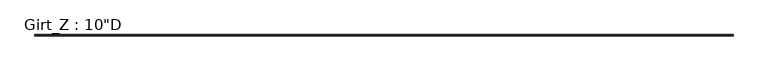
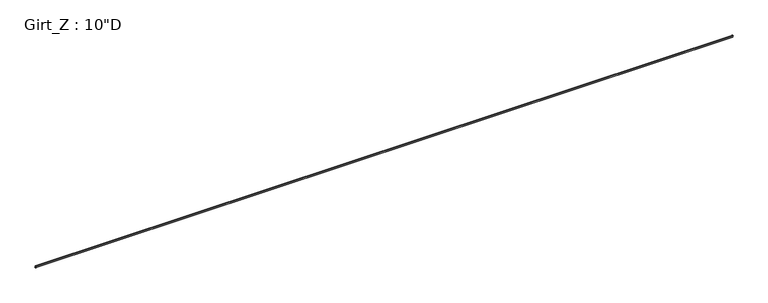
"""IFC4 building model written with IfcOpenShell, lengths in millimetres: beam geometry."""

from ifc_helpers import new_model, si_unit, point, frame, frame_2d, origin, place, context, project, spatial, polyline, circle_curve, trimmed, segment, composite_curve, outline, extrude, source, transform, mapped, element, save


def beam_261beed4(model_context):
    return source(origin(), model_context, "Body", "SweptSolid", [
        extrude(outline(composite_curve([segment(polyline([(-77.9859375, 127.0), (-3.3734375, 127.0)]), True, "CONTINUOUS"), segment(trimmed(circle_curve(frame_2d((-3.3734375, 122.2375)), 4.7625), [point((-3.3734375, 127.0))], [point((1.3890625, 122.2375))], False, "CARTESIAN"), True, "CONTINUOUS"), segment(polyline([(1.3890625, 122.2375), (1.3890625, -122.2389339)]), True, "CONTINUOUS"), segment(trimmed(circle_curve(frame_2d((3.3748024, -122.2389339)), 1.9857399), [point((1.3890625, -122.2389339))], [point((3.2694106, -124.221875))], True, "CARTESIAN"), True, "CONTINUOUS"), segment(polyline([(3.2694106, -124.221875), (83.0404765, -124.221875), (94.4528742, -110.621109), (96.5810415, -112.4068534), (84.3359375, -127.0), (-1.3890625, -127.0), (-1.3890625, 122.2381931)]), True, "CONTINUOUS"), segment(trimmed(circle_curve(frame_2d((-3.3741066, 122.2381931)), 1.9850441), [point((-1.3890625, 122.2381931))], [point((-3.3005807, 124.221875))], True, "CARTESIAN"), True, "CONTINUOUS"), segment(polyline([(-3.3005807, 124.221875), (-76.6904765, 124.221875), (-88.1028742, 110.621109), (-90.2310415, 112.4068534), (-77.9859375, 127.0)]), True, "CONTINUOUS")], self_intersect=False)), frame((-44323.0, 0.0, 0.0), z_axis=(1.0, 0.0, 0.0), x_axis=(0.0, 1.0, 0.0)), (0.0, 0.0, 1.0), 88430.1),
    ])


if __name__ == "__main__":
    model = new_model("IFC4")
    model_context = context("Model", 3, world=origin())
    ifc_project = project(units=[si_unit("LENGTHUNIT", "METRE", prefix="MILLI")], contexts=[model_context])
    site = spatial("IfcSite", under=ifc_project)
    building = spatial("IfcBuilding", under=site)
    placement = place(None, origin())
    beam_shape = beam_261beed4(model_context)
    element("IfcBeam", 1, ObjectType="Girt_Z : 10\"D", at=placement, inside=building, context=model_context, shape_type="MappedRepresentation", body=[
        mapped(beam_shape, transform((0.0, 0.0, 0.0), x_axis=(1.0, 0.0, 0.0), y_axis=(0.0, 1.0, 0.0), z_axis=(0.0, 0.0, 1.0))),
    ])
    save(model, "model.ifc")

# Revit data of these elements
# Type "Girt_Z : 10\"D"
#   half leg = 0' - 1 11/16"
#   Web_Thickness = 0' - 0 7/64"
#   Length [instance default] = 10' - 0"
#   Leg_2 = 0' - 3 3/8"
#   Leg_1 = 0' - 3 1/8"
#   Height = 0' - 10"
#   Structural Material [instance default] = none
# Element 1 (IfcBeam, "Girt_Z : 10\"D")
#   Structural Material = STRUCTURAL STEEL - SEE STRUCT. DWGS
#   Materials on its faces: "STRUCTURAL STEEL - SEE STRUCT. DWGS"
# Materials
#   "STRUCTURAL STEEL - SEE STRUCT. DWGS": class "Metal", colour RGB 137 146 153, transparency 0, Description = "Steel, mill finish", Cost = 0
